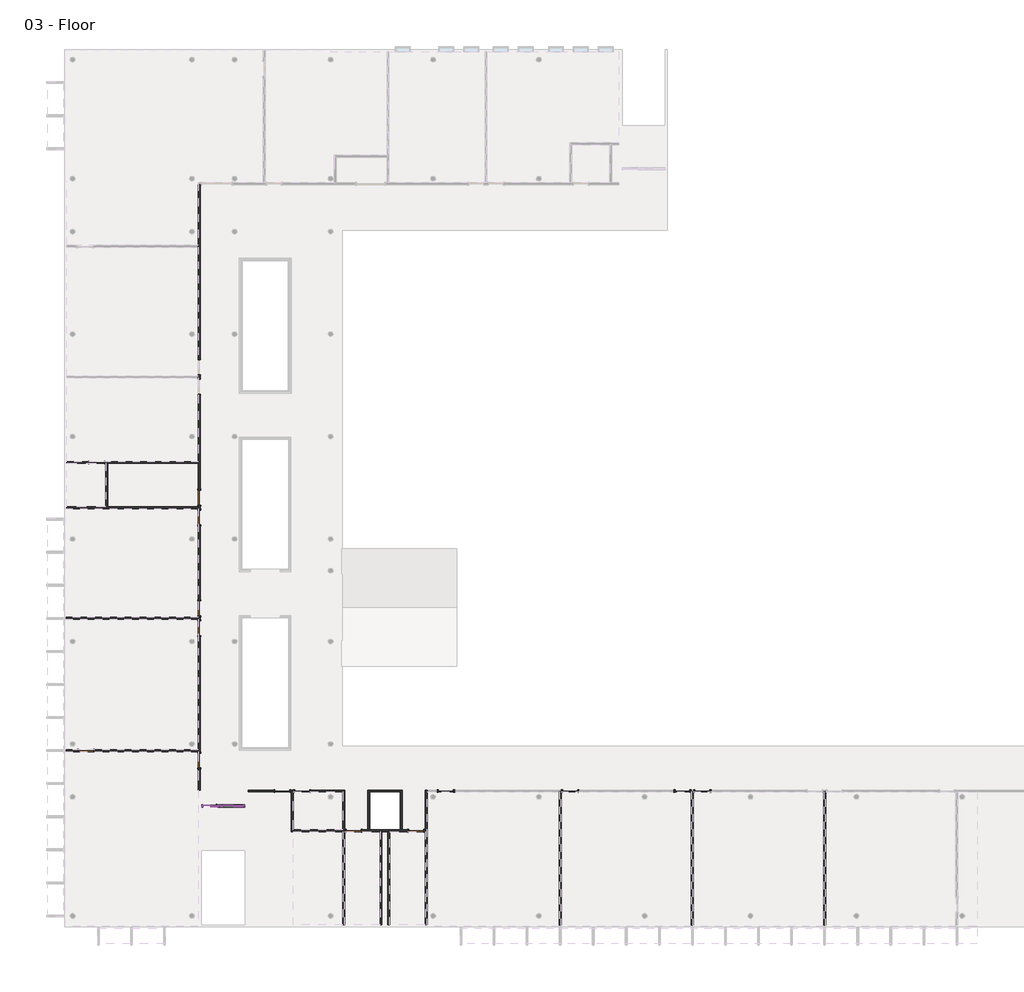
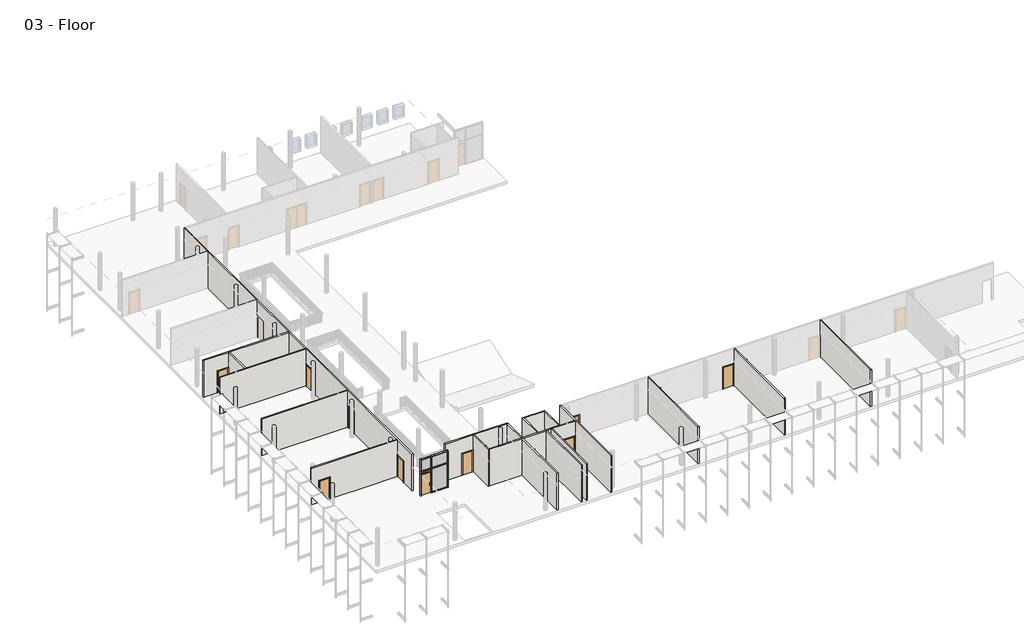
# One storey, part 1 of 4: 19 walls, 18 members, 16 doors, 4 plates.
"""IFC4 building model written with IfcOpenShell, lengths in millimetres."""

import ifcopenshell
import ifcopenshell.guid

model = None  # the IFC model being written
_history = None  # IfcOwnerHistory: only IFC2X3 demands one
_inside = {}  # id of a spatial element -> (the spatial element, [elements in it])
_under = {}  # id of a project, library or spatial element -> (it, [spatial elements below it])
_declared = {}  # id of a project -> (the project, [libraries it declares])
_typed = {}  # id of a type object -> (the type object, [elements of that type])
_made_of = {}  # id of a material, layer set ... -> (it, [elements and type objects made of it])


def new_model(schema):
    """Start an empty IFC model of exactly this schema.

    Asked for "IFC4X3", IfcOpenShell would pick the latest addendum, in which some entities
    have other attributes; the version numbers below select the first issue.
    IFC2X3 requires an IfcOwnerHistory on every rooted entity: one is made here for all.
    """
    global model, _history
    if schema == "IFC4X3":
        model = ifcopenshell.file(schema_version=(4, 3, 0, 0))
    else:
        model = ifcopenshell.file(schema=schema)
    _inside.clear()
    _under.clear()
    _declared.clear()
    _typed.clear()
    _made_of.clear()
    _history = None
    if model.schema == "IFC2X3":
        org = make("IfcOrganization", Name="unknown")
        user = make(
            "IfcPersonAndOrganization",
            ThePerson=make("IfcPerson", FamilyName="unknown"),
            TheOrganization=org,
        )
        app = make(
            "IfcApplication",
            ApplicationDeveloper=org,
            Version="unknown",
            ApplicationFullName="unknown",
            ApplicationIdentifier="unknown",
        )
        _history = make(
            "IfcOwnerHistory",
            OwningUser=user,
            OwningApplication=app,
            ChangeAction="ADDED",
            CreationDate=0,
        )
    return model


def make(cls, **values):
    """One entity of the class cls with the attributes given. An attribute that is None is left unset."""
    return model.create_entity(
        cls, **{name: value for name, value in values.items() if value is not None}
    )


def rooted(cls, **values):
    """An entity with a GlobalId (a new one), such as an element, a storey or a relation."""
    return make(cls, GlobalId=ifcopenshell.guid.new(), OwnerHistory=_history, **values)


def si_unit(unit_type, name, prefix=None):
    """IfcSIUnit, for example si_unit("LENGTHUNIT", "METRE", prefix="MILLI")."""
    return make("IfcSIUnit", UnitType=unit_type, Prefix=prefix, Name=name)


def assignment(units):
    """IfcUnitAssignment: the units of a project."""
    return None if units is None else make("IfcUnitAssignment", Units=units)


def point(xyz):
    """IfcCartesianPoint."""
    return None if xyz is None else make("IfcCartesianPoint", Coordinates=xyz)


def direction(xyz):
    """IfcDirection."""
    return None if xyz is None else make("IfcDirection", DirectionRatios=xyz)


def frame(location, z_axis=None, x_axis=None):
    """IfcAxis2Placement3D, a coordinate frame: its origin and axes. An axis left out is left unset."""
    return make(
        "IfcAxis2Placement3D",
        Location=point(location),
        Axis=direction(z_axis),
        RefDirection=direction(x_axis),
    )


def origin():
    """The frame at (0, 0, 0) with its axes left unset."""
    return frame((0.0, 0.0, 0.0))


def origin_with_axes():
    """The frame at (0, 0, 0) with the z axis (0, 0, 1) and the x axis (1, 0, 0) written out."""
    return frame((0.0, 0.0, 0.0), z_axis=(0.0, 0.0, 1.0), x_axis=(1.0, 0.0, 0.0))


def place(relative_to, where):
    """IfcLocalPlacement: puts the frame where relative to a parent placement (None: the world)."""
    return make(
        "IfcLocalPlacement", PlacementRelTo=relative_to, RelativePlacement=where
    )


def context(
    kind, dimensions, precision=None, world=None, true_north=None, identifier=None
):
    """IfcGeometricRepresentationContext, for example the 3D "Model" context."""
    return make(
        "IfcGeometricRepresentationContext",
        ContextIdentifier=identifier,
        ContextType=kind,
        CoordinateSpaceDimension=dimensions,
        Precision=precision,
        WorldCoordinateSystem=world,
        TrueNorth=true_north,
    )


def project(units=None, contexts=None):
    """IfcProject with its units and contexts."""
    return rooted(
        "IfcProject",
        Name="project",
        RepresentationContexts=contexts,
        UnitsInContext=assignment(units),
    )


def spatial(cls, under=None, at=None, **own):
    """A site, building, storey or space (cls), placed at a placement, below another one or the project."""
    s = rooted(cls, ObjectPlacement=at, **own)
    if under is not None:
        _under.setdefault(under.id(), (under, []))[1].append(s)
    return s


def polyline(points):
    """IfcPolyline through the points."""
    return make("IfcPolyline", Points=[point(p) for p in points])


def outline(outer, holes=None, kind="AREA"):
    """IfcArbitraryClosedProfileDef: a profile drawn as a closed curve; with holes, ...WithVoids."""
    if holes is None:
        return make("IfcArbitraryClosedProfileDef", ProfileType=kind, OuterCurve=outer)
    return make(
        "IfcArbitraryProfileDefWithVoids",
        ProfileType=kind,
        OuterCurve=outer,
        InnerCurves=holes,
    )


def extrude(swept, where, along, depth):
    """IfcExtrudedAreaSolid: the profile swept, set in the frame where, extruded along a direction by depth."""
    return make(
        "IfcExtrudedAreaSolid",
        SweptArea=swept,
        Position=where,
        ExtrudedDirection=direction(along),
        Depth=depth,
    )


def faces_of(points, faces, orient=None, outer=None):
    """IfcFace entities. A face is a list of loops; a loop is a list of indices into points, from 0.

    orient and outer hold one flag for each loop. By default every Orientation is true, the
    first loop of a face is its IfcFaceOuterBound and the others are IfcFaceBound.
    """
    made = []
    for i, loops in enumerate(faces):
        bounds = []
        for j, loop in enumerate(loops):
            is_outer = j == 0 if outer is None else outer[i][j]
            bounds.append(
                make(
                    "IfcFaceOuterBound" if is_outer else "IfcFaceBound",
                    Bound=make("IfcPolyLoop", Polygon=[points[k] for k in loop]),
                    Orientation=True if orient is None else orient[i][j],
                )
            )
        made.append(make("IfcFace", Bounds=bounds))
    return made


def faceted_brep(points, faces, orient=None, outer=None, voids=None):
    """IfcFacetedBrep: a solid bounded by flat faces; with voids (closed shells), ...WithVoids."""
    shared = [point(p) for p in points]
    hull = make("IfcClosedShell", CfsFaces=faces_of(shared, faces, orient, outer))
    if voids is None:
        return make("IfcFacetedBrep", Outer=hull)
    return make(
        "IfcFacetedBrepWithVoids",
        Outer=hull,
        Voids=[
            make(cls, CfsFaces=faces_of(shared, fs, o, b)) for cls, fs, o, b in voids
        ],
    )


def shape(context_of_items, identifier, shape_type, items):
    """IfcShapeRepresentation: the items that make up one representation, for example the "Body"."""
    return make(
        "IfcShapeRepresentation",
        ContextOfItems=context_of_items,
        RepresentationIdentifier=identifier,
        RepresentationType=shape_type,
        Items=items,
    )


def source(mapping_origin, context_of_items, identifier, shape_type, items):
    """IfcRepresentationMap: a shape defined once, which mapped items show again and again."""
    return make(
        "IfcRepresentationMap",
        MappingOrigin=mapping_origin,
        MappedRepresentation=shape(context_of_items, identifier, shape_type, items),
    )


def transform(
    local_origin,
    x_axis=None,
    y_axis=None,
    z_axis=None,
    scale=None,
    scale2=None,
    scale3=None,
    uniform=True,
):
    """IfcCartesianTransformationOperator3D, or its non-uniform kind. x_axis, y_axis, z_axis: its Axis1, 2, 3."""
    if uniform:
        return make(
            "IfcCartesianTransformationOperator3D",
            Axis1=direction(x_axis),
            Axis2=direction(y_axis),
            LocalOrigin=point(local_origin),
            Scale=scale,
            Axis3=direction(z_axis),
        )
    return make(
        "IfcCartesianTransformationOperator3DnonUniform",
        Axis1=direction(x_axis),
        Axis2=direction(y_axis),
        LocalOrigin=point(local_origin),
        Scale=scale,
        Axis3=direction(z_axis),
        Scale2=scale2,
        Scale3=scale3,
    )


def mapped(mapping_source, mapping_target):
    """IfcMappedItem: shows the shape of a source again, moved by a transform."""
    return make(
        "IfcMappedItem", MappingSource=mapping_source, MappingTarget=mapping_target
    )


def made_of(thing, what):
    """Note that an element or type object is made of a material, layer set ...; save() writes the relation."""
    if what is not None:
        _made_of.setdefault(what.id(), (what, []))[1].append(thing)
    return thing


def element(
    cls,
    number,
    at=None,
    inside=None,
    cuts=None,
    type_object=None,
    material=None,
    context=None,
    identifier="Body",
    shape_type=None,
    held_by="IfcProductDefinitionShape",
    body=None,
    shapes=None,
    **own,
):
    """One element of the class cls, such as IfcWall. Its Tag is "e" and its number.

    at: its placement. inside: the storey or other place that contains it. cuts: it is an
    opening in that element (IfcRelVoidsElement). A single representation is given by context,
    identifier, shape_type and body (its items); several are given by shapes. held_by: the class
    of the entity that holds the representations. save() writes the other relations.
    """
    e = rooted(cls, Tag="e%d" % number, ObjectPlacement=at, **own)
    if body is not None:
        shapes = [shape(context, identifier, shape_type, body)]
    if shapes is not None:
        e.Representation = make(held_by, Representations=shapes)
    if inside is not None:
        _inside.setdefault(inside.id(), (inside, []))[1].append(e)
    if cuts is not None:
        rooted(
            "IfcRelVoidsElement", RelatingBuildingElement=cuts, RelatedOpeningElement=e
        )
    if type_object is not None:
        _typed.setdefault(type_object.id(), (type_object, []))[1].append(e)
    return made_of(e, material)


def aggregate(whole, parts):
    """IfcRelAggregates: a whole, such as a stair, and the parts it consists of."""
    return rooted("IfcRelAggregates", RelatingObject=whole, RelatedObjects=parts)


def save(model, path):
    """Write the relations noted so far, then the file.

    IfcRelAggregates (storeys below a building ...), IfcRelContainedInSpatialStructure (elements
    in a storey), IfcRelDefinesByType, IfcRelAssociatesMaterial and IfcRelDeclares: one each for
    every whole, place, type object, material and project.
    """
    for whole, parts in _under.values():
        aggregate(whole, parts)
    for where, things in _inside.values():
        rooted(
            "IfcRelContainedInSpatialStructure",
            RelatedElements=things,
            RelatingStructure=where,
        )
    for kind, things in _typed.values():
        rooted("IfcRelDefinesByType", RelatedObjects=things, RelatingType=kind)
    for what, things in _made_of.values():
        rooted("IfcRelAssociatesMaterial", RelatedObjects=things, RelatingMaterial=what)
    for by, libraries in _declared.values():
        rooted("IfcRelDeclares", RelatingContext=by, RelatedDefinitions=libraries)
    model.write(path)


def curtain_wall_sgl_glass_curtain_wall_sgl_glass_c2d4b377(model_context):
    return source(origin(), model_context, "Body", "SweptSolid", [
        extrude(outline(polyline([(-355.6, 12.7), (-355.6, -38.1), (-381.0, -38.1), (-381.0, 12.7), (-355.6, 12.7)])), frame((0.0, 0.0, 762.0), z_axis=(0.0, 0.0, 1.0), x_axis=(1.0, 0.0, 0.0)), (0.0, 0.0, 1.0), 228.6),
        extrude(outline(polyline([(-381.0, -101.6), (-381.0, -50.8), (-355.6, -50.8), (-355.6, -101.6), (-381.0, -101.6)])), frame((0.0, 0.0, 762.0), z_axis=(0.0, 0.0, 1.0), x_axis=(1.0, 0.0, 0.0)), (0.0, 0.0, 1.0), 228.6),
        extrude(outline(polyline([(457.2, -50.8), (-457.2, -50.8), (-457.2, -38.1), (457.2, -38.1), (457.2, -50.8)])), origin_with_axes(), (0.0, 0.0, 1.0), 2133.6),
    ])


def door_305aa2a5(model_context):
    return source(origin(), model_context, "Body", "SweptSolid", [
        extrude(outline(polyline([(2209.8, -533.4), (0.0, -533.4), (0.0, -457.2), (2133.6, -457.2), (2133.6, 457.2), (0.0, 457.2), (0.0, 533.4), (2209.8, 533.4), (2209.8, -533.4)])), frame((0.0, -82.55, 0.0), z_axis=(0.0, 1.0, 0.0), x_axis=(0.0, 0.0, 1.0)), (0.0, 0.0, 1.0), 25.4),
        extrude(outline(polyline([(2209.8, 533.4), (2209.8, -533.4), (0.0, -533.4), (0.0, -457.2), (2133.6, -457.2), (2133.6, 457.2), (0.0, 457.2), (0.0, 533.4), (2209.8, 533.4)])), frame((0.0, 57.15, 0.0), z_axis=(0.0, 1.0, 0.0), x_axis=(0.0, 0.0, 1.0)), (0.0, 0.0, 1.0), 25.4),
        extrude(outline(polyline([(457.2, -6.35), (457.2, -57.15), (-457.2, -57.15), (-457.2, -6.35), (457.2, -6.35)])), origin_with_axes(), (0.0, 0.0, 1.0), 2133.6),
    ])


def door_e5f9f3c4(model_context):
    return source(origin(), model_context, "Body", "SweptSolid", [
        extrude(outline(polyline([(2209.8, -533.4), (0.0, -533.4), (0.0, -457.2), (2133.6, -457.2), (2133.6, 457.2), (0.0, 457.2), (0.0, 533.4), (2209.8, 533.4), (2209.8, -533.4)])), frame((0.0, 57.15, 0.0), z_axis=(0.0, 1.0, 0.0), x_axis=(0.0, 0.0, 1.0)), (0.0, 0.0, 1.0), 25.4),
        extrude(outline(polyline([(2209.8, 533.4), (2209.8, -533.4), (0.0, -533.4), (0.0, -457.2), (2133.6, -457.2), (2133.6, 457.2), (0.0, 457.2), (0.0, 533.4), (2209.8, 533.4)])), frame((0.0, -82.55, 0.0), z_axis=(0.0, 1.0, 0.0), x_axis=(0.0, 0.0, 1.0)), (0.0, 0.0, 1.0), 25.4),
        extrude(outline(polyline([(457.2, 6.35), (-457.2, 6.35), (-457.2, 57.15), (457.2, 57.15), (457.2, 6.35)])), origin_with_axes(), (0.0, 0.0, 1.0), 2133.6),
    ])


def member_2b49869a(model_context):
    return source(origin(), model_context, "Body", "SweptSolid", [
        extrude(outline(polyline([(31.75, 63.5), (31.75, -63.5), (-31.75, -63.5), (-31.75, 63.5), (31.75, 63.5)])), frame((0.0, 0.0, -1219.2), z_axis=(0.0, 0.0, 1.0), x_axis=(1.0, 0.0, 0.0)), (0.0, 0.0, 1.0), 1219.2),
    ])


def member_75074519(model_context):
    return source(origin(), model_context, "Body", "SweptSolid", [
        extrude(outline(polyline([(0.0, 63.5), (0.0, -63.5), (-63.5, -63.5), (-63.5, 63.5), (0.0, 63.5)])), frame((0.0, 0.0, -1219.2), z_axis=(0.0, 0.0, 1.0), x_axis=(1.0, 0.0, 0.0)), (0.0, 0.0, 1.0), 1219.2),
    ])


def member_6186cc23(model_context):
    return source(origin(), model_context, "Body", "SweptSolid", [
        extrude(outline(polyline([(31.75, 63.5), (31.75, -63.5), (-31.75, -63.5), (-31.75, 63.5), (31.75, 63.5)])), frame((0.0, 0.0, -2165.35), z_axis=(0.0, 0.0, 1.0), x_axis=(1.0, 0.0, 0.0)), (0.0, 0.0, 1.0), 2165.35),
    ])


def member_5d67b9fc(model_context):
    return source(origin(), model_context, "Body", "SweptSolid", [
        extrude(outline(polyline([(31.75, 63.5), (31.75, -63.5), (-31.75, -63.5), (-31.75, 63.5), (31.75, 63.5)])), frame((0.0, 0.0, -273.05), z_axis=(0.0, 0.0, 1.0), x_axis=(1.0, 0.0, 0.0)), (0.0, 0.0, 1.0), 273.05),
    ])


def member_c327c56d(model_context):
    return source(origin(), model_context, "Body", "SweptSolid", [
        extrude(outline(polyline([(0.0, 63.5), (0.0, -63.5), (-63.5, -63.5), (-63.5, 63.5), (0.0, 63.5)])), frame((0.0, 0.0, -273.05), z_axis=(0.0, 0.0, 1.0), x_axis=(1.0, 0.0, 0.0)), (0.0, 0.0, 1.0), 273.05),
    ])


def member_a50b3cda(model_context):
    return source(origin(), model_context, "Body", "SweptSolid", [
        extrude(outline(polyline([(0.0, 63.5), (0.0, -63.5), (-63.5, -63.5), (-63.5, 63.5), (0.0, 63.5)])), frame((0.0, 0.0, -2165.35), z_axis=(0.0, 0.0, 1.0), x_axis=(1.0, 0.0, 0.0)), (0.0, 0.0, 1.0), 2165.35),
    ])


def member_410c6227(model_context):
    return source(origin(), model_context, "Body", "SweptSolid", [
        extrude(outline(polyline([(31.75, 63.5), (31.75, -63.5), (-31.75, -63.5), (-31.75, 63.5), (31.75, 63.5)])), frame((0.0, 0.0, -914.4), z_axis=(0.0, 0.0, 1.0), x_axis=(1.0, 0.0, 0.0)), (0.0, 0.0, 1.0), 914.4),
    ])


def member_73c23c35(model_context):
    return source(origin(), model_context, "Body", "SweptSolid", [
        extrude(outline(polyline([(0.0, 63.5), (0.0, -63.5), (-63.5, -63.5), (-63.5, 63.5), (0.0, 63.5)])), frame((0.0, 0.0, -914.4), z_axis=(0.0, 0.0, 1.0), x_axis=(1.0, 0.0, 0.0)), (0.0, 0.0, 1.0), 914.4),
    ])


def member_59c53a79(model_context):
    return source(origin(), model_context, "Body", "SweptSolid", [
        extrude(outline(polyline([(0.0, 63.5), (0.0, -63.5), (-63.5, -63.5), (-63.5, 63.5), (0.0, 63.5)])), frame((0.0, 0.0, -1245.39375), z_axis=(0.0, 0.0, 1.0), x_axis=(1.0, 0.0, 0.0)), (0.0, 0.0, 1.0), 1245.39375),
    ])


def member_c46932f7(model_context):
    return source(origin(), model_context, "Body", "SweptSolid", [
        extrude(outline(polyline([(31.75, 63.5), (31.75, -63.5), (-31.75, -63.5), (-31.75, 63.5), (31.75, 63.5)])), frame((0.0, 0.0, -1245.39375), z_axis=(0.0, 0.0, 1.0), x_axis=(1.0, 0.0, 0.0)), (0.0, 0.0, 1.0), 1245.39375),
    ])


def member_40e8ea34(model_context):
    return source(origin(), model_context, "Body", "SweptSolid", [
        extrude(outline(polyline([(31.75, 63.5), (31.75, -63.5), (-31.75, -63.5), (-31.75, 63.5), (31.75, 63.5)])), frame((0.0, 0.0, -267.49375), z_axis=(0.0, 0.0, 1.0), x_axis=(1.0, 0.0, 0.0)), (0.0, 0.0, 1.0), 267.49375),
    ])


def member_f5b3432e(model_context):
    return source(origin(), model_context, "Body", "SweptSolid", [
        extrude(outline(polyline([(0.0, 63.5), (0.0, -63.5), (-63.5, -63.5), (-63.5, 63.5), (0.0, 63.5)])), frame((0.0, 0.0, -267.49375), z_axis=(0.0, 0.0, 1.0), x_axis=(1.0, 0.0, 0.0)), (0.0, 0.0, 1.0), 267.49375),
    ])


def system_panel_glazed_8dc8626f(model_context):
    return source(origin(), model_context, "Body", "SweptSolid", [
        extrude(outline(polyline([(457.2, -44.45), (-457.2, -44.45), (-457.2, -19.05), (457.2, -19.05), (457.2, -44.45)])), origin_with_axes(), (0.0, 0.0, 1.0), 209.55),
    ])


def system_panel_glazed_2e5f6ce9(model_context):
    return source(origin(), model_context, "Body", "SweptSolid", [
        extrude(outline(polyline([(457.2, -44.45), (-457.2, -44.45), (-457.2, -19.05), (457.2, -19.05), (457.2, -44.45)])), origin_with_axes(), (0.0, 0.0, 1.0), 1123.95),
    ])


def system_panel_glazed_8d3e4aee(model_context):
    return source(origin(), model_context, "Body", "SweptSolid", [
        extrude(outline(polyline([(0.0, -756.44375), (0.0, 488.95), (0.0, 756.44375), (2101.85, 756.44375), (2343.15, 756.44375), (2343.15, 488.95), (2343.15, -756.44375), (2101.85, -756.44375), (0.0, -756.44375)])), frame((0.0, -44.45, 0.0), z_axis=(0.0, 1.0, 0.0), x_axis=(0.0, 0.0, 1.0)), (0.0, 0.0, 1.0), 25.4),
    ])


def system_panel_glazed_fabe228a(model_context):
    return source(origin(), model_context, "Body", "SweptSolid", [
        extrude(outline(polyline([(0.0, -756.44375), (0.0, 488.95), (0.0, 756.44375), (1123.95, 756.44375), (1123.95, 488.95), (1123.95, -756.44375), (0.0, -756.44375)])), frame((0.0, -44.45, 0.0), z_axis=(0.0, 1.0, 0.0), x_axis=(0.0, 0.0, 1.0)), (0.0, 0.0, 1.0), 25.4),
    ])


model = new_model("IFC4")

# Units and contexts
model_context = context("Model", 3, world=origin())
ifc_project = project(units=[si_unit("LENGTHUNIT", "METRE", prefix="MILLI")], contexts=[model_context])

# Site, building, storey
site = spatial("IfcSite", under=ifc_project)
building = spatial("IfcBuilding", under=site)
storey = spatial("IfcBuildingStorey", under=building, Name="03 - Floor", Elevation=7315.2)

# Doors
placement = place(None, origin())
curtain_wall_sgl_glass_curtain_wall_sgl_glass_shape = curtain_wall_sgl_glass_curtain_wall_sgl_glass_c2d4b377(model_context)
element("IfcDoor", 1, ObjectType="Curtain Wall Sgl Glass : Curtain Wall Sgl Glass", at=placement, inside=storey, context=model_context, shape_type="MappedRepresentation", body=[
    mapped(curtain_wall_sgl_glass_curtain_wall_sgl_glass_shape, transform((9097.2957476, 7356.4, 7315.2), x_axis=(-1.0, 0.0, 0.0), y_axis=(0.0, -1.0, 0.0), z_axis=(0.0, 0.0, 1.0))),
])
door_shape = door_305aa2a5(model_context)
element("IfcDoor", 2, ObjectType="Single-Flush : 36\" x 84\"", at=placement, inside=storey, context=model_context, shape_type="MappedRepresentation", body=[
    mapped(door_shape, transform((21743.3207476, 5832.4, 7315.2), x_axis=(1.0, 0.0, 0.0), y_axis=(0.0, 1.0, 0.0), z_axis=(0.0, 0.0, 1.0))),
])
element("IfcDoor", 3, ObjectType="Single-Flush : 36\" x 84\"", at=placement, inside=storey, context=model_context, shape_type="MappedRepresentation", body=[
    mapped(door_shape, transform((2109.1207476, 28463.8, 7315.2), x_axis=(1.0, 0.0, 0.0), y_axis=(0.0, 1.0, 0.0), z_axis=(0.0, 0.0, 1.0))),
])
element("IfcDoor", 4, ObjectType="Single-Flush : 36\" x 84\"", at=placement, inside=storey, context=model_context, shape_type="MappedRepresentation", body=[
    mapped(door_shape, transform((8414.6707476, 26304.8, 7315.2), x_axis=(0.0, -1.0, 0.0), y_axis=(1.0, 0.0, 0.0), z_axis=(0.0, 0.0, 1.0))),
])
element("IfcDoor", 5, ObjectType="Single-Flush : 36\" x 84\"", at=placement, inside=storey, context=model_context, shape_type="MappedRepresentation", body=[
    mapped(door_shape, transform((8414.6707476, 19497.6, 7315.2), x_axis=(0.0, -1.0, 0.0), y_axis=(1.0, 0.0, 0.0), z_axis=(0.0, 0.0, 1.0))),
])
element("IfcDoor", 6, ObjectType="Single-Flush : 36\" x 84\"", at=placement, inside=storey, context=model_context, shape_type="MappedRepresentation", body=[
    mapped(door_shape, transform((13513.7207476, 8277.15, 7315.2), x_axis=(1.0, 0.0, 0.0), y_axis=(0.0, 1.0, 0.0), z_axis=(0.0, 0.0, 1.0))),
])
element("IfcDoor", 7, ObjectType="Single-Flush : 36\" x 84\"", at=placement, inside=storey, context=model_context, shape_type="MappedRepresentation", body=[
    mapped(door_shape, transform((38113.6207476, 8277.15, 7315.2), x_axis=(1.0, 0.0, 0.0), y_axis=(0.0, 1.0, 0.0), z_axis=(0.0, 0.0, 1.0))),
])
door_2_shape = door_e5f9f3c4(model_context)
element("IfcDoor", 8, ObjectType="Single-Flush : 36\" x 84\"", at=placement, inside=storey, context=model_context, shape_type="MappedRepresentation", body=[
    mapped(door_2_shape, transform((17907.9207476, 5832.4, 7315.2), x_axis=(-1.0, 0.0, 0.0), y_axis=(0.0, -1.0, 0.0), z_axis=(0.0, 0.0, 1.0))),
])
element("IfcDoor", 9, ObjectType="Single-Flush : 36\" x 84\"", at=placement, inside=storey, context=model_context, shape_type="MappedRepresentation", body=[
    mapped(door_2_shape, transform((8414.6707476, 25085.6, 7315.2), x_axis=(0.0, 1.0, 0.0), y_axis=(-1.0, 0.0, 0.0), z_axis=(0.0, 0.0, 1.0))),
])
element("IfcDoor", 10, ObjectType="Single-Flush : 36\" x 84\"", at=placement, inside=storey, context=model_context, shape_type="MappedRepresentation", body=[
    mapped(door_2_shape, transform((8414.6707476, 18278.4, 7315.2), x_axis=(0.0, 1.0, 0.0), y_axis=(-1.0, 0.0, 0.0), z_axis=(0.0, 0.0, 1.0))),
])
element("IfcDoor", 11, ObjectType="Single-Flush : 36\" x 84\"", at=placement, inside=storey, context=model_context, shape_type="MappedRepresentation", body=[
    mapped(door_2_shape, transform((1448.7207476, 10760.0, 7315.2), x_axis=(-1.0, 0.0, 0.0), y_axis=(0.0, -1.0, 0.0), z_axis=(0.0, 0.0, 1.0))),
])
element("IfcDoor", 12, ObjectType="Single-Flush : 36\" x 84\"", at=placement, inside=storey, context=model_context, shape_type="MappedRepresentation", body=[
    mapped(door_2_shape, transform((8414.6707476, 10150.4, 7315.2), x_axis=(0.0, 1.0, 0.0), y_axis=(-1.0, 0.0, 0.0), z_axis=(0.0, 0.0, 1.0))),
])
element("IfcDoor", 13, ObjectType="Single-Flush : 36\" x 84\"", at=placement, inside=storey, context=model_context, shape_type="MappedRepresentation", body=[
    mapped(door_2_shape, transform((14732.9207476, 8277.15, 7315.2), x_axis=(-1.0, 0.0, 0.0), y_axis=(0.0, -1.0, 0.0), z_axis=(0.0, 0.0, 1.0))),
])
element("IfcDoor", 14, ObjectType="Single-Flush : 36\" x 84\"", at=placement, inside=storey, context=model_context, shape_type="MappedRepresentation", body=[
    mapped(door_2_shape, transform((23572.1207476, 8277.15, 7315.2), x_axis=(-1.0, 0.0, 0.0), y_axis=(0.0, -1.0, 0.0), z_axis=(0.0, 0.0, 1.0))),
])
element("IfcDoor", 15, ObjectType="Single-Flush : 36\" x 84\"", at=placement, inside=storey, context=model_context, shape_type="MappedRepresentation", body=[
    mapped(door_2_shape, transform((31204.8207476, 8277.15, 7315.2), x_axis=(-1.0, 0.0, 0.0), y_axis=(0.0, -1.0, 0.0), z_axis=(0.0, 0.0, 1.0))),
])
element("IfcDoor", 16, ObjectType="Single-Flush : 36\" x 84\"", at=placement, inside=storey, context=model_context, shape_type="MappedRepresentation", body=[
    mapped(door_2_shape, transform((39332.8207476, 8277.15, 7315.2), x_axis=(-1.0, 0.0, 0.0), y_axis=(0.0, -1.0, 0.0), z_axis=(0.0, 0.0, 1.0))),
])

# Members
member_shape = member_2b49869a(model_context)
element("IfcMember", 17, ObjectType="Rectangular Mullion : 2.5\" x 5\" rectangular", at=placement, inside=storey, context=model_context, shape_type="MappedRepresentation", body=[
    mapped(member_shape, transform((9586.2457476, 7356.4, 9753.6), x_axis=(-1.0, 0.0, 0.0), y_axis=(0.0, 1.0, 0.0), z_axis=(0.0, 0.0, -1.0))),
])
member_2_shape = member_75074519(model_context)
element("IfcMember", 18, ObjectType="Rectangular Mullion : 2.5\" x 5\" rectangular", at=placement, inside=storey, context=model_context, shape_type="MappedRepresentation", body=[
    mapped(member_2_shape, transform((11194.3832476, 7356.4, 10972.8), x_axis=(1.0, 0.0, 0.0), y_axis=(0.0, 1.0, 0.0), z_axis=(0.0, 0.0, 1.0))),
])
element("IfcMember", 19, ObjectType="Rectangular Mullion : 2.5\" x 5\" rectangular", at=placement, inside=storey, context=model_context, shape_type="MappedRepresentation", body=[
    mapped(member_2_shape, transform((8576.5957476, 7356.4, 9753.6), x_axis=(-1.0, 0.0, 0.0), y_axis=(0.0, 1.0, 0.0), z_axis=(0.0, 0.0, -1.0))),
])
member_3_shape = member_6186cc23(model_context)
element("IfcMember", 20, ObjectType="Rectangular Mullion : 2.5\" x 5\" rectangular", at=placement, inside=storey, context=model_context, shape_type="MappedRepresentation", body=[
    mapped(member_3_shape, transform((9586.2457476, 7356.4, 7315.2), x_axis=(-1.0, 0.0, 0.0), y_axis=(0.0, 1.0, 0.0), z_axis=(0.0, 0.0, -1.0))),
])
member_4_shape = member_5d67b9fc(model_context)
element("IfcMember", 21, ObjectType="Rectangular Mullion : 2.5\" x 5\" rectangular", at=placement, inside=storey, context=model_context, shape_type="MappedRepresentation", body=[
    mapped(member_4_shape, transform((9586.2457476, 7356.4, 9480.55), x_axis=(-1.0, 0.0, 0.0), y_axis=(0.0, 1.0, 0.0), z_axis=(0.0, 0.0, -1.0))),
])
member_5_shape = member_c327c56d(model_context)
element("IfcMember", 22, ObjectType="Rectangular Mullion : 2.5\" x 5\" rectangular", at=placement, inside=storey, context=model_context, shape_type="MappedRepresentation", body=[
    mapped(member_5_shape, transform((11194.3832476, 7356.4, 9753.6), x_axis=(1.0, 0.0, 0.0), y_axis=(0.0, 1.0, 0.0), z_axis=(0.0, 0.0, 1.0))),
])
member_6_shape = member_a50b3cda(model_context)
element("IfcMember", 23, ObjectType="Rectangular Mullion : 2.5\" x 5\" rectangular", at=placement, inside=storey, context=model_context, shape_type="MappedRepresentation", body=[
    mapped(member_6_shape, transform((11194.3832476, 7356.4, 9480.55), x_axis=(1.0, 0.0, 0.0), y_axis=(0.0, 1.0, 0.0), z_axis=(0.0, 0.0, 1.0))),
])
member_7_shape = member_410c6227(model_context)
element("IfcMember", 24, ObjectType="Rectangular Mullion : 2.5\" x 5\" rectangular", at=placement, inside=storey, context=model_context, shape_type="MappedRepresentation", body=[
    mapped(member_7_shape, transform((8640.0957476, 7356.4, 9753.6), x_axis=(0.0, 0.0, 1.0), y_axis=(0.0, 1.0, 0.0), z_axis=(-1.0, 0.0, 0.0))),
])
element("IfcMember", 25, ObjectType="Rectangular Mullion : 2.5\" x 5\" rectangular", at=placement, inside=storey, context=model_context, shape_type="MappedRepresentation", body=[
    mapped(member_7_shape, transform((8640.0957476, 7356.4, 9480.55), x_axis=(0.0, 0.0, 1.0), y_axis=(0.0, 1.0, 0.0), z_axis=(-1.0, 0.0, 0.0))),
])
member_8_shape = member_73c23c35(model_context)
element("IfcMember", 26, ObjectType="Rectangular Mullion : 2.5\" x 5\" rectangular", at=placement, inside=storey, context=model_context, shape_type="MappedRepresentation", body=[
    mapped(member_8_shape, transform((8640.0957476, 7356.4, 10972.8), x_axis=(0.0, 0.0, 1.0), y_axis=(0.0, 1.0, 0.0), z_axis=(-1.0, 0.0, 0.0))),
])
element("IfcMember", 27, ObjectType="Rectangular Mullion : 2.5\" x 5\" rectangular", at=placement, inside=storey, context=model_context, shape_type="MappedRepresentation", body=[
    mapped(member_6_shape, transform((8576.5957476, 7356.4, 7315.2), x_axis=(-1.0, 0.0, 0.0), y_axis=(0.0, 1.0, 0.0), z_axis=(0.0, 0.0, -1.0))),
])
element("IfcMember", 28, ObjectType="Rectangular Mullion : 2.5\" x 5\" rectangular", at=placement, inside=storey, context=model_context, shape_type="MappedRepresentation", body=[
    mapped(member_5_shape, transform((8576.5957476, 7356.4, 9480.55), x_axis=(-1.0, 0.0, 0.0), y_axis=(0.0, 1.0, 0.0), z_axis=(0.0, 0.0, -1.0))),
])
member_9_shape = member_59c53a79(model_context)
element("IfcMember", 29, ObjectType="Rectangular Mullion : 2.5\" x 5\" rectangular", at=placement, inside=storey, context=model_context, shape_type="MappedRepresentation", body=[
    mapped(member_9_shape, transform((11130.8832476, 7356.4, 7315.2), x_axis=(0.0, 0.0, -1.0), y_axis=(0.0, 1.0, 0.0), z_axis=(1.0, 0.0, 0.0))),
])
member_10_shape = member_c46932f7(model_context)
element("IfcMember", 30, ObjectType="Rectangular Mullion : 2.5\" x 5\" rectangular", at=placement, inside=storey, context=model_context, shape_type="MappedRepresentation", body=[
    mapped(member_10_shape, transform((9885.4894976, 7356.4, 9753.6), x_axis=(0.0, 0.0, 1.0), y_axis=(0.0, 1.0, 0.0), z_axis=(-1.0, 0.0, 0.0))),
])
element("IfcMember", 31, ObjectType="Rectangular Mullion : 2.5\" x 5\" rectangular", at=placement, inside=storey, context=model_context, shape_type="MappedRepresentation", body=[
    mapped(member_9_shape, transform((9885.4894976, 7356.4, 10972.8), x_axis=(0.0, 0.0, 1.0), y_axis=(0.0, 1.0, 0.0), z_axis=(-1.0, 0.0, 0.0))),
])
member_11_shape = member_40e8ea34(model_context)
element("IfcMember", 32, ObjectType="Rectangular Mullion : 2.5\" x 5\" rectangular", at=placement, inside=storey, context=model_context, shape_type="MappedRepresentation", body=[
    mapped(member_11_shape, transform((9617.9957476, 7356.4, 9753.6), x_axis=(0.0, 0.0, 1.0), y_axis=(0.0, 1.0, 0.0), z_axis=(-1.0, 0.0, 0.0))),
])
member_12_shape = member_f5b3432e(model_context)
element("IfcMember", 33, ObjectType="Rectangular Mullion : 2.5\" x 5\" rectangular", at=placement, inside=storey, context=model_context, shape_type="MappedRepresentation", body=[
    mapped(member_12_shape, transform((9617.9957476, 7356.4, 10972.8), x_axis=(0.0, 0.0, 1.0), y_axis=(0.0, 1.0, 0.0), z_axis=(-1.0, 0.0, 0.0))),
])
element("IfcMember", 34, ObjectType="Rectangular Mullion : 2.5\" x 5\" rectangular", at=placement, inside=storey, context=model_context, shape_type="MappedRepresentation", body=[
    mapped(member_12_shape, transform((9885.4894976, 7356.4, 7315.2), x_axis=(0.0, 0.0, -1.0), y_axis=(0.0, 1.0, 0.0), z_axis=(1.0, 0.0, 0.0))),
])

# Plates
system_panel_glazed_shape = system_panel_glazed_8dc8626f(model_context)
element("IfcPlate", 35, ObjectType="System Panel : Glazed", at=placement, inside=storey, context=model_context, shape_type="MappedRepresentation", body=[
    mapped(system_panel_glazed_shape, transform((9097.2957476, 7356.4, 9512.3), x_axis=(-1.0, 0.0, 0.0), y_axis=(0.0, -1.0, 0.0), z_axis=(0.0, 0.0, 1.0))),
])
system_panel_glazed_2_shape = system_panel_glazed_2e5f6ce9(model_context)
element("IfcPlate", 36, ObjectType="System Panel : Glazed", at=placement, inside=storey, context=model_context, shape_type="MappedRepresentation", body=[
    mapped(system_panel_glazed_2_shape, transform((9097.2957476, 7356.4, 9785.35), x_axis=(-1.0, 0.0, 0.0), y_axis=(0.0, -1.0, 0.0), z_axis=(0.0, 0.0, 1.0))),
])
system_panel_glazed_3_shape = system_panel_glazed_8d3e4aee(model_context)
element("IfcPlate", 37, ObjectType="System Panel : Glazed", at=placement, inside=storey, context=model_context, shape_type="MappedRepresentation", body=[
    mapped(system_panel_glazed_3_shape, transform((10374.4394976, 7356.4, 7378.7), x_axis=(-1.0, 0.0, 0.0), y_axis=(0.0, -1.0, 0.0), z_axis=(0.0, 0.0, 1.0))),
])
system_panel_glazed_4_shape = system_panel_glazed_fabe228a(model_context)
element("IfcPlate", 38, ObjectType="System Panel : Glazed", at=placement, inside=storey, context=model_context, shape_type="MappedRepresentation", body=[
    mapped(system_panel_glazed_4_shape, transform((10374.4394976, 7356.4, 9785.35), x_axis=(-1.0, 0.0, 0.0), y_axis=(0.0, -1.0, 0.0), z_axis=(0.0, 0.0, 1.0))),
])

# Walls
element("IfcWall", 39, ObjectType="Typ. Partition Wall", at=placement, inside=storey, context=model_context, shape_type="Brep", body=[
    faceted_brep([(8357.5207476, 17821.2, 7315.2), (8357.5207476, 10817.15, 7315.2), (8357.5207476, 10702.85, 7315.2), (8357.5207476, 10607.6, 7315.2), (8357.5207476, 10607.6, 9448.8), (8357.5207476, 9693.2, 9448.8), (8357.5207476, 9693.2, 7315.2), (8357.5207476, 8334.3, 7315.2), (8357.5207476, 8334.3, 10972.8), (8357.5207476, 10702.85, 10972.8), (8357.5207476, 10817.15, 10972.8), (8357.5207476, 18830.85, 10972.8), (8357.5207476, 18945.15, 10972.8), (8357.5207476, 25638.05, 10972.8), (8357.5207476, 25752.35, 10972.8), (8357.5207476, 28406.65, 10972.8), (8357.5207476, 28520.95, 10972.8), (8357.5207476, 33664.45, 10972.8), (8357.5207476, 33778.75, 10972.8), (8357.5207476, 41690.85, 10972.8), (8357.5207476, 41805.15, 10972.8), (8357.5207476, 45545.3, 10972.8), (8357.5207476, 45545.3, 7315.2), (8357.5207476, 41805.15, 7315.2), (8357.5207476, 41690.85, 7315.2), (8357.5207476, 34788.4, 7315.2), (8357.5207476, 34788.4, 9448.8), (8357.5207476, 33874.0, 9448.8), (8357.5207476, 33874.0, 7315.2), (8357.5207476, 33778.75, 7315.2), (8357.5207476, 33664.45, 7315.2), (8357.5207476, 33569.2, 7315.2), (8357.5207476, 33569.2, 9448.8), (8357.5207476, 32654.8, 9448.8), (8357.5207476, 32654.8, 7315.2), (8357.5207476, 28520.95, 7315.2), (8357.5207476, 28406.65, 7315.2), (8357.5207476, 26762.0, 7315.2), (8357.5207476, 26762.0, 9448.8), (8357.5207476, 25847.6, 9448.8), (8357.5207476, 25847.6, 7315.2), (8357.5207476, 25752.35, 7315.2), (8357.5207476, 25638.05, 7315.2), (8357.5207476, 25542.8, 7315.2), (8357.5207476, 25542.8, 9448.8), (8357.5207476, 24628.4, 9448.8), (8357.5207476, 24628.4, 7315.2), (8357.5207476, 19954.8, 7315.2), (8357.5207476, 19954.8, 9448.8), (8357.5207476, 19040.4, 9448.8), (8357.5207476, 19040.4, 7315.2), (8357.5207476, 18945.15, 7315.2), (8357.5207476, 18830.85, 7315.2), (8357.5207476, 18735.6, 7315.2), (8357.5207476, 18735.6, 9448.8), (8357.5207476, 17821.2, 9448.8), (8471.8207476, 10607.6, 9448.8), (8471.8207476, 10607.6, 7315.2), (8471.8207476, 17821.2, 7315.2), (8471.8207476, 17821.2, 9448.8), (8471.8207476, 18735.6, 9448.8), (8471.8207476, 18735.6, 7315.2), (8471.8207476, 19040.4, 7315.2), (8471.8207476, 19040.4, 9448.8), (8471.8207476, 19954.8, 9448.8), (8471.8207476, 19954.8, 7315.2), (8471.8207476, 24628.4, 7315.2), (8471.8207476, 24628.4, 9448.8), (8471.8207476, 25542.8, 9448.8), (8471.8207476, 25542.8, 7315.2), (8471.8207476, 25847.6, 7315.2), (8471.8207476, 25847.6, 9448.8), (8471.8207476, 26762.0, 9448.8), (8471.8207476, 26762.0, 7315.2), (8471.8207476, 32654.8, 7315.2), (8471.8207476, 32654.8, 9448.8), (8471.8207476, 33569.2, 9448.8), (8471.8207476, 33569.2, 7315.2), (8471.8207476, 33874.0, 7315.2), (8471.8207476, 33874.0, 9448.8), (8471.8207476, 34788.4, 9448.8), (8471.8207476, 34788.4, 7315.2), (8471.8207476, 45545.3, 7315.2), (8471.8207476, 45545.3, 10972.8), (8471.8207476, 8334.3, 10972.8), (8471.8207476, 8334.3, 7315.2), (8471.8207476, 9693.2, 7315.2), (8471.8207476, 9693.2, 9448.8)], [[[0, 1, 2, 3, 4, 5, 6, 7, 8, 9, 10, 11, 12, 13, 14, 15, 16, 17, 18, 19, 20, 21, 22, 23, 24, 25, 26, 27, 28, 29, 30, 31, 32, 33, 34, 35, 36, 37, 38, 39, 40, 41, 42, 43, 44, 45, 46, 47, 48, 49, 50, 51, 52, 53, 54, 55]], [[56, 57, 58, 59, 60, 61, 62, 63, 64, 65, 66, 67, 68, 69, 70, 71, 72, 73, 74, 75, 76, 77, 78, 79, 80, 81, 82, 83, 84, 85, 86, 87]], [[78, 77, 31, 30, 29, 28]], [[25, 24, 23, 22, 82, 81]], [[70, 69, 43, 42, 41, 40]], [[37, 36, 35, 34, 74, 73]], [[62, 61, 53, 52, 51, 50]], [[47, 46, 66, 65]], [[58, 57, 3, 2, 1, 0]], [[86, 85, 7, 6]], [[8, 7, 85, 84]], [[21, 20, 19, 18, 17, 16, 15, 14, 13, 12, 11, 10, 9, 8, 84, 83]], [[22, 21, 83, 82]], [[79, 78, 28, 27]], [[80, 79, 27, 26]], [[81, 80, 26, 25]], [[32, 31, 77, 76]], [[33, 32, 76, 75]], [[34, 33, 75, 74]], [[71, 70, 40, 39]], [[72, 71, 39, 38]], [[73, 72, 38, 37]], [[44, 43, 69, 68]], [[45, 44, 68, 67]], [[46, 45, 67, 66]], [[63, 62, 50, 49]], [[64, 63, 49, 48]], [[65, 64, 48, 47]], [[54, 53, 61, 60]], [[55, 54, 60, 59]], [[0, 55, 59, 58]], [[4, 3, 57, 56]], [[5, 4, 56, 87]], [[6, 5, 87, 86]]]),
])
element("IfcWall", 40, ObjectType="Typ. Partition Wall", at=placement, inside=storey, context=model_context, shape_type="Brep", body=[
    faceted_brep([(13970.9207476, 8220.0, 7315.2), (14066.1707476, 8220.0, 7315.2), (14180.4707476, 8220.0, 7315.2), (14275.7207476, 8220.0, 7315.2), (14275.7207476, 8220.0, 9448.8), (15190.1207476, 8220.0, 9448.8), (15190.1207476, 8220.0, 7315.2), (17241.1707476, 8220.0, 7315.2), (17355.4707476, 8220.0, 7315.2), (17355.4707476, 8220.0, 10972.8), (17241.1707476, 8220.0, 10972.8), (14180.4707476, 8220.0, 10972.8), (14066.1707476, 8220.0, 10972.8), (11413.4582476, 8220.0, 10972.8), (11413.4582476, 8220.0, 7315.2), (13056.5207476, 8220.0, 7315.2), (13056.5207476, 8220.0, 9448.8), (13970.9207476, 8220.0, 9448.8), (14275.7207476, 8334.3, 9448.8), (14275.7207476, 8334.3, 7315.2), (13970.9207476, 8334.3, 7315.2), (13970.9207476, 8334.3, 9448.8), (13056.5207476, 8334.3, 9448.8), (13056.5207476, 8334.3, 7315.2), (11413.4582476, 8334.3, 7315.2), (11413.4582476, 8334.3, 10972.8), (17355.4707476, 8334.3, 10972.8), (17355.4707476, 8334.3, 7315.2), (15190.1207476, 8334.3, 7315.2), (15190.1207476, 8334.3, 9448.8)], [[[0, 1, 2, 3, 4, 5, 6, 7, 8, 9, 10, 11, 12, 13, 14, 15, 16, 17]], [[18, 19, 20, 21, 22, 23, 24, 25, 26, 27, 28, 29]], [[20, 19, 3, 2, 1, 0]], [[15, 14, 24, 23]], [[28, 27, 8, 7, 6]], [[13, 12, 11, 10, 9, 26, 25]], [[9, 8, 27, 26]], [[14, 13, 25, 24]], [[21, 20, 0, 17]], [[22, 21, 17, 16]], [[23, 22, 16, 15]], [[4, 3, 19, 18]], [[5, 4, 18, 29]], [[6, 5, 29, 28]]]),
])
element("IfcWall", 41, ObjectType="Typ. Partition Wall", at=placement, inside=storey, context=model_context, shape_type="Brep", body=[
    faceted_brep([(14180.4707476, 5775.25, 7315.2), (14180.4707476, 5889.55, 7315.2), (14180.4707476, 8220.0, 7315.2), (14180.4707476, 8220.0, 10972.8), (14180.4707476, 5889.55, 10972.8), (14180.4707476, 5775.25, 10972.8), (14066.1707476, 5775.25, 7315.2), (14066.1707476, 5775.25, 10972.8), (14066.1707476, 8220.0, 10972.8), (14066.1707476, 8220.0, 7315.2)], [[[0, 1, 2, 3, 4, 5]], [[6, 7, 8, 9]], [[2, 1, 0, 6, 9]], [[5, 4, 3, 8, 7]], [[0, 5, 7, 6]], [[3, 2, 9, 8]]]),
])
element("IfcWall", 42, ObjectType="Typ. Partition Wall", at=placement, inside=storey, context=model_context, shape_type="Brep", body=[
    faceted_brep([(17355.4707476, 53.9, 7315.2), (17355.4707476, 5775.25, 7315.2), (17355.4707476, 5889.55, 7315.2), (17355.4707476, 8220.0, 7315.2), (17355.4707476, 8220.0, 10972.8), (17355.4707476, 5889.55, 10972.8), (17355.4707476, 5775.25, 10972.8), (17355.4707476, 53.9, 10972.8), (17241.1707476, 53.9, 7315.2), (17241.1707476, 53.9, 10972.8), (17241.1707476, 5775.25, 10972.8), (17241.1707476, 5889.55, 10972.8), (17241.1707476, 8220.0, 10972.8), (17241.1707476, 8220.0, 7315.2), (17241.1707476, 5889.55, 7315.2), (17241.1707476, 5775.25, 7315.2)], [[[0, 1, 2, 3, 4, 5, 6, 7]], [[8, 9, 10, 11, 12, 13, 14, 15]], [[3, 2, 1, 0, 8, 15, 14, 13]], [[7, 6, 5, 4, 12, 11, 10, 9]], [[0, 7, 9, 8]], [[4, 3, 13, 12]]]),
])
element("IfcWall", 43, ObjectType="Typ. Partition Wall", at=placement, inside=storey, context=model_context, shape_type="Brep", body=[
    faceted_brep([(17450.7207476, 5775.25, 7315.2), (17450.7207476, 5775.25, 9448.8), (18365.1207476, 5775.25, 9448.8), (18365.1207476, 5775.25, 7315.2), (19527.1707476, 5775.25, 7315.2), (19641.4707476, 5775.25, 7315.2), (20009.7707476, 5775.25, 7315.2), (20124.0707476, 5775.25, 7315.2), (21286.1207476, 5775.25, 7315.2), (21286.1207476, 5775.25, 9448.8), (22200.5207476, 5775.25, 9448.8), (22200.5207476, 5775.25, 7315.2), (22308.4707476, 5775.25, 7315.2), (22308.4707476, 5775.25, 10972.8), (20124.0707476, 5775.25, 10972.8), (20009.7707476, 5775.25, 10972.8), (19641.4707476, 5775.25, 10972.8), (19527.1707476, 5775.25, 10972.8), (17355.4707476, 5775.25, 10972.8), (17355.4707476, 5775.25, 7315.2), (17450.7207476, 5889.55, 9448.8), (17450.7207476, 5889.55, 7315.2), (17355.4707476, 5889.55, 7315.2), (17355.4707476, 5889.55, 10972.8), (18765.1707476, 5889.55, 10972.8), (18879.4707476, 5889.55, 10972.8), (20771.7707476, 5889.55, 10972.8), (20886.0707476, 5889.55, 10972.8), (22308.4707476, 5889.55, 10972.8), (22308.4707476, 5889.55, 7315.2), (22200.5207476, 5889.55, 7315.2), (22200.5207476, 5889.55, 9448.8), (21286.1207476, 5889.55, 9448.8), (21286.1207476, 5889.55, 7315.2), (20886.0707476, 5889.55, 7315.2), (20771.7707476, 5889.55, 7315.2), (18879.4707476, 5889.55, 7315.2), (18765.1707476, 5889.55, 7315.2), (18365.1207476, 5889.55, 7315.2), (18365.1207476, 5889.55, 9448.8)], [[[0, 1, 2, 3, 4, 5, 6, 7, 8, 9, 10, 11, 12, 13, 14, 15, 16, 17, 18, 19]], [[20, 21, 22, 23, 24, 25, 26, 27, 28, 29, 30, 31, 32, 33, 34, 35, 36, 37, 38, 39]], [[21, 0, 19, 22]], [[3, 38, 37, 36, 35, 34, 33, 8, 7, 6, 5, 4]], [[11, 30, 29, 12]], [[13, 28, 27, 26, 25, 24, 23, 18, 17, 16, 15, 14]], [[1, 0, 21, 20]], [[2, 1, 20, 39]], [[3, 2, 39, 38]], [[31, 30, 11, 10]], [[32, 31, 10, 9]], [[33, 32, 9, 8]], [[13, 12, 29, 28]], [[19, 18, 23, 22]]]),
    faceted_brep([(14180.4707476, 5775.25, 10972.8), (14180.4707476, 5775.25, 7315.2), (17241.1707476, 5775.25, 7315.2), (17241.1707476, 5775.25, 10972.8), (14180.4707476, 5889.55, 7315.2), (14180.4707476, 5889.55, 10972.8), (17241.1707476, 5889.55, 10972.8), (17241.1707476, 5889.55, 7315.2)], [[[0, 1, 2, 3]], [[4, 5, 6, 7]], [[1, 4, 7, 2]], [[5, 0, 3, 6]], [[1, 0, 5, 4]], [[3, 2, 7, 6]]]),
])
element("IfcWall", 44, ObjectType="Typ. Partition Wall", at=placement, inside=storey, context=model_context, shape_type="SweptSolid", body=[
    extrude(outline(polyline([(19527.1707476, 53.9), (19527.1707476, 5775.25), (19641.4707476, 5775.25), (19641.4707476, 53.9), (19527.1707476, 53.9)])), frame((0.0, 0.0, 7315.2), z_axis=(0.0, 0.0, 1.0), x_axis=(1.0, 0.0, 0.0)), (0.0, 0.0, 1.0), 3657.6),
])
element("IfcWall", 45, ObjectType="Typ. Partition Wall", at=placement, inside=storey, context=model_context, shape_type="SweptSolid", body=[
    extrude(outline(polyline([(20009.7707476, 53.9), (20009.7707476, 5775.25), (20124.0707476, 5775.25), (20124.0707476, 53.9), (20009.7707476, 53.9)])), frame((0.0, 0.0, 7315.2), z_axis=(0.0, 0.0, 1.0), x_axis=(1.0, 0.0, 0.0)), (0.0, 0.0, 1.0), 3657.6),
])
element("IfcWall", 46, ObjectType="Typ. Partition Wall", at=placement, inside=storey, context=model_context, shape_type="Brep", body=[
    faceted_brep([(18879.4707476, 5889.55, 7315.2), (18879.4707476, 8220.0, 7315.2), (18879.4707476, 8334.3, 7315.2), (18879.4707476, 8334.3, 10972.8), (18879.4707476, 8220.0, 10972.8), (18879.4707476, 5889.55, 10972.8), (18765.1707476, 5889.55, 7315.2), (18765.1707476, 5889.55, 10972.8), (18765.1707476, 8334.3, 10972.8), (18765.1707476, 8334.3, 7315.2)], [[[0, 1, 2, 3, 4, 5]], [[6, 7, 8, 9]], [[2, 1, 0, 6, 9]], [[5, 4, 3, 8, 7]], [[3, 2, 9, 8]], [[0, 5, 7, 6]]]),
])
element("IfcWall", 47, ObjectType="Typ. Partition Wall", at=placement, inside=storey, context=model_context, shape_type="Brep", body=[
    faceted_brep([(20886.0707476, 5889.55, 7315.2), (20886.0707476, 8334.3, 7315.2), (20886.0707476, 8334.3, 10972.8), (20886.0707476, 5889.55, 10972.8), (20771.7707476, 5889.55, 7315.2), (20771.7707476, 5889.55, 10972.8), (20771.7707476, 8220.0, 10972.8), (20771.7707476, 8334.3, 10972.8), (20771.7707476, 8334.3, 7315.2), (20771.7707476, 8220.0, 7315.2)], [[[0, 1, 2, 3]], [[4, 5, 6, 7, 8, 9]], [[1, 0, 4, 9, 8]], [[3, 2, 7, 6, 5]], [[2, 1, 8, 7]], [[0, 3, 5, 4]]]),
])
element("IfcWall", 48, ObjectType="Typ. Partition Wall", at=placement, inside=storey, context=model_context, shape_type="Brep", body=[
    faceted_brep([(22422.7707476, 53.9, 7315.2), (22422.7707476, 8220.0, 7315.2), (22422.7707476, 8334.3, 7315.2), (22422.7707476, 8334.3, 10972.8), (22422.7707476, 8220.0, 10972.8), (22422.7707476, 53.9, 10972.8), (22308.4707476, 53.9, 7315.2), (22308.4707476, 53.9, 10972.8), (22308.4707476, 5775.25, 10972.8), (22308.4707476, 5889.55, 10972.8), (22308.4707476, 8334.3, 10972.8), (22308.4707476, 8334.3, 7315.2), (22308.4707476, 5889.55, 7315.2), (22308.4707476, 5775.25, 7315.2)], [[[0, 1, 2, 3, 4, 5]], [[6, 7, 8, 9, 10, 11, 12, 13]], [[2, 1, 0, 6, 13, 12, 11]], [[5, 4, 3, 10, 9, 8, 7]], [[3, 2, 11, 10]], [[0, 5, 7, 6]]]),
])
element("IfcWall", 49, ObjectType="Typ. Partition Wall", at=placement, inside=storey, context=model_context, shape_type="SweptSolid", body=[
    extrude(outline(polyline([(20771.7707476, 8220.0), (18879.4707476, 8220.0), (18879.4707476, 8334.3), (20771.7707476, 8334.3), (20771.7707476, 8220.0)])), frame((0.0, 0.0, 7315.2), z_axis=(0.0, 0.0, 1.0), x_axis=(1.0, 0.0, 0.0)), (0.0, 0.0, 1.0), 3657.6),
])
element("IfcWall", 50, ObjectType="Typ. Partition Wall", at=placement, inside=storey, context=model_context, shape_type="Brep", body=[
    faceted_brep([(280.3207476, 25638.05, 7315.2), (8357.5207476, 25638.05, 7315.2), (8357.5207476, 25638.05, 10972.8), (280.3207476, 25638.05, 10972.8), (280.3207476, 25752.35, 7315.2), (280.3207476, 25752.35, 10972.8), (2661.5707476, 25752.35, 10972.8), (2775.8707476, 25752.35, 10972.8), (8357.5207476, 25752.35, 10972.8), (8357.5207476, 25752.35, 7315.2), (2775.8707476, 25752.35, 7315.2), (2661.5707476, 25752.35, 7315.2)], [[[0, 1, 2, 3]], [[4, 5, 6, 7, 8, 9, 10, 11]], [[1, 0, 4, 11, 10, 9]], [[0, 3, 5, 4]], [[2, 1, 9, 8]], [[3, 2, 8, 7, 6, 5]]]),
])
element("IfcWall", 51, ObjectType="Typ. Partition Wall", at=placement, inside=storey, context=model_context, shape_type="SweptSolid", body=[
    extrude(outline(polyline([(7315.2, 242.2207476), (7315.2, 8357.5207476), (10972.8, 8357.5207476), (10972.8, 280.3207476), (10972.8, 242.2207476), (7315.2, 242.2207476)])), frame((0.0, 18830.85, 0.0), z_axis=(0.0, 1.0, 0.0), x_axis=(0.0, 0.0, 1.0)), (0.0, 0.0, 1.0), 114.3),
])
element("IfcWall", 52, ObjectType="Typ. Partition Wall", at=placement, inside=storey, context=model_context, shape_type="SweptSolid", body=[
    extrude(outline(polyline([(7315.2, 242.2207476), (7315.2, 991.5207476), (9448.8, 991.5207476), (9448.8, 1905.9207476), (7315.2, 1905.9207476), (7315.2, 8357.5207476), (10972.8, 8357.5207476), (10972.8, 280.3207476), (10972.8, 242.2207476), (7315.2, 242.2207476)])), frame((0.0, 10702.85, 0.0), z_axis=(0.0, 1.0, 0.0), x_axis=(0.0, 0.0, 1.0)), (0.0, 0.0, 1.0), 114.3),
])
element("IfcWall", 53, ObjectType="Typ. Partition Wall", at=placement, inside=storey, context=model_context, shape_type="Brep", body=[
    faceted_brep([(2566.3207476, 28406.65, 9448.8), (2566.3207476, 28406.65, 7315.2), (2661.5707476, 28406.65, 7315.2), (2775.8707476, 28406.65, 7315.2), (8357.5207476, 28406.65, 7315.2), (8357.5207476, 28406.65, 10972.8), (2775.8707476, 28406.65, 10972.8), (2661.5707476, 28406.65, 10972.8), (280.3207476, 28406.65, 10972.8), (280.3207476, 28406.65, 7315.2), (1651.9207476, 28406.65, 7315.2), (1651.9207476, 28406.65, 9448.8), (8357.5207476, 28520.95, 7315.2), (2566.3207476, 28520.95, 7315.2), (2566.3207476, 28520.95, 9448.8), (1651.9207476, 28520.95, 9448.8), (1651.9207476, 28520.95, 7315.2), (280.3207476, 28520.95, 7315.2), (280.3207476, 28520.95, 10972.8), (8357.5207476, 28520.95, 10972.8)], [[[0, 1, 2, 3, 4, 5, 6, 7, 8, 9, 10, 11]], [[12, 13, 14, 15, 16, 17, 18, 19]], [[4, 3, 2, 1, 13, 12]], [[10, 9, 17, 16]], [[9, 8, 18, 17]], [[5, 4, 12, 19]], [[8, 7, 6, 5, 19, 18]], [[14, 13, 1, 0]], [[15, 14, 0, 11]], [[16, 15, 11, 10]]]),
])
element("IfcWall", 54, ObjectType="Typ. Partition Wall", at=placement, inside=storey, context=model_context, shape_type="SweptSolid", body=[
    extrude(outline(polyline([(2775.8707476, 28406.65), (2775.8707476, 25752.35), (2661.5707476, 25752.35), (2661.5707476, 28406.65), (2775.8707476, 28406.65)])), frame((0.0, 0.0, 7315.2), z_axis=(0.0, 0.0, 1.0), x_axis=(1.0, 0.0, 0.0)), (0.0, 0.0, 1.0), 3657.6),
])
element("IfcWall", 55, ObjectType="Typ. Partition Wall", at=placement, inside=storey, context=model_context, shape_type="SweptSolid", body=[
    extrude(outline(polyline([(15.8, 7315.2), (15.8, 10972.8), (53.9, 10972.8), (8220.0, 10972.8), (8220.0, 7315.2), (15.8, 7315.2)])), frame((46794.0707476, 0.0, 0.0), z_axis=(1.0, 0.0, 0.0), x_axis=(0.0, 1.0, 0.0)), (0.0, 0.0, 1.0), 114.3),
])
element("IfcWall", 56, ObjectType="Typ. Partition Wall", at=placement, inside=storey, context=model_context, shape_type="SweptSolid", body=[
    extrude(outline(polyline([(15.8, 7315.2), (15.8, 10972.8), (53.9, 10972.8), (8220.0, 10972.8), (8220.0, 7315.2), (15.8, 7315.2)])), frame((38666.0707476, 0.0, 0.0), z_axis=(1.0, 0.0, 0.0), x_axis=(0.0, 1.0, 0.0)), (0.0, 0.0, 1.0), 114.3),
])
element("IfcWall", 57, ObjectType="Typ. Partition Wall", at=placement, inside=storey, context=model_context, shape_type="SweptSolid", body=[
    extrude(outline(polyline([(15.8, 7315.2), (15.8, 10972.8), (53.9, 10972.8), (8220.0, 10972.8), (8220.0, 7315.2), (15.8, 7315.2)])), frame((30538.0707476, 0.0, 0.0), z_axis=(1.0, 0.0, 0.0), x_axis=(0.0, 1.0, 0.0)), (0.0, 0.0, 1.0), 114.3),
])

save(model, "model.ifc")

# Revit data of these elements
# Project information
#   built-in parameter 1006321 = "Issue Date"
#   built-in parameter 1006320 = "Project Status"
#   built-in parameter 1006319 = "Owner"
#   built-in parameter 1006318 = "Enter address here"
#   built-in parameter 1006317 = "Project Name"
#   built-in parameter 1006316 = "Project Number"
# Grids (mm)
#   "1": line (635.921, -2868.377) -> (635.921, 59109.339)
#   "2": line (10592.721, -2868.377) -> (10592.721, 59109.339)
#   "3": line (16485.521, -2868.377) -> (16485.521, 59109.339)
#   "4": line (22784.721, -2868.377) -> (22784.721, 59109.339)
#   "5": line (29287.121, -2868.377) -> (29287.121, 59109.339)
#   "6": line (35789.521, -2868.377) -> (35789.521, 59109.339)
#   "7": line (42291.921, -2868.377) -> (42291.921, 13344.021)
#   "8": line (48794.321, -2868.377) -> (48794.321, 13344.021)
#   "9": line (55296.721, -2868.377) -> (55296.721, 13344.021)
#   "10": line (66066.321, 13344.021) -> (66066.321, -2868.377)
#   "A": line (-3253.24, 53228.8) -> (38986.476, 53228.8)
#   "B": line (-3253.24, 45913.6) -> (38986.476, 45913.6)
#   "C": line (-3253.24, 42662.4) -> (38986.476, 42662.4)
#   "D": line (-3253.24, 36363.2) -> (20075.346, 36363.2)
#   "E": line (-3253.24, 30064) -> (20075.346, 30064)
#   "F": line (-3253.24, 23764.8) -> (20075.346, 23764.8)
#   "G": line (-3253.24, 17465.6) -> (25935.992, 17465.6)
#   "H": line (-3253.24, 11166.4) -> (68405.099, 11166.4)
#   "I": line (-3253.24, 7915.2) -> (68405.099, 7915.2)
#   "J": line (-3253.24, 600) -> (68405.099, 600)
#   "1.1": line (7951.121, -2868.377) -> (7951.121, 59109.339)
#   "F.1": line (-3253.24, 21821.7) -> (25935.992, 21821.7)
# Type "Curtain Wall Sgl Glass : Curtain Wall Sgl Glass"
#   Assembly Code = "B2030100"
#   Offset = 0' - 2"
#   Function = 1
#   Handle Material = Metal - Aluminum
#   Glazing Material = Glass
# Type "Single-Flush : 36\" x 84\""
#   Type Mark = "1"
#   Assembly Code = "C1020"
#   Thickness = 0' - 2"
#   Height = 7' - 0"
#   Trim Projection Ext = 0' - 1"
#   Trim Projection Int = 0' - 1"
#   Trim Width = 0' - 3"
#   Width = 3' - 0"
#   Function = 0
#   Door Material = Door - Panel
#   Frame Material = Door - Frame
#   Wall Closure = (empty or 0)
# Type "Rectangular Mullion : 2.5\" x 5\" rectangular"
#   built-in parameter 1007304 = 0.416667 (stored number, unit not read)
#   built-in parameter 1007301 = 0.104167 (stored number, unit not read)
#   built-in parameter 1007300 = 0.104167 (stored number, unit not read)
# Type "Typ. Partition Wall"
#   Assembly Code = "B2010"
#   Type Mark = "A1"
#   Width = 0' - 4 1/2"
#   Layers, outside or top first: 0' - 0 1/2" "Gypsum Wall Board" (function 1); 0' - 3 1/2" "Metal - Stud Layer" (function 1); 0' - 0 1/2" "Gypsum Wall Board" (function 1)
# Element 1 (IfcDoor, "Curtain Wall Sgl Glass : Curtain Wall Sgl Glass")
#   Frame Material = "Alum."
#   Frame Type = "1"
#   Phase Created = New Construction
#   Materials on its faces: "Metal - Aluminum", "Glass"
# Elements 2, 3, 4, 5, 6, 7, 8, 9, 10, 11, 12, 13, 14, 15, 16 (IfcDoor, "Single-Flush : 36\" x 84\"")
#   Frame Material = "Wood"
#   Frame Type = "3"
#   Phase Created = New Construction
#   Materials on its faces: "Door - Frame", "Door - Panel"
# Elements 17, 18, 19, 20, 21, 22, 23, 24, 25, 26, 27, 28, 29, 30, 31, 32, 33, 34 (IfcMember, "Rectangular Mullion : 2.5\" x 5\" rectangular")
#   Phase Created = New Construction
#   Materials on its faces: "Metal - Aluminum"
# Elements 35, 36, 37, 38 (IfcPlate, "System Panel : Glazed")
#   Phase Created = New Construction
#   Materials on its faces: "Glass"
# Elements 39, 40, 42, 43, 44, 45, 49, 50, 51, 52, 53, 54, 55, 56, 57 (IfcWall, "Typ. Partition Wall")
#   Top Offset = 0' - 0"
#   Base Offset = 0' - 0"
#   wall height = 12' - 0"
#   Phase Created = New Construction
#   Base Constraint = 03 - Floor
#   Top Constraint = Roof
#   Materials on its faces: "Default Wall", "Gypsum Wall Board"
# Elements 41, 46, 47, 48 (IfcWall, "Typ. Partition Wall")
#   Top Offset = 0' - 0"
#   Base Offset = 0' - 0"
#   wall height = 12' - 0"
#   Phase Created = New Construction
#   Base Constraint = 03 - Floor
#   Top Constraint = Roof
#   Materials on its faces: "Gypsum Wall Board", "Default Wall"
# Materials
#   "Metal - Aluminum": class "Metal", colour RGB 140 140 140, transparency 0
#   "Glass": class "Glass", colour RGB 0 128 192, transparency 0.75
#   "Door - Panel": class "Wood", colour RGB 210 159 95, transparency 0
#   "Door - Frame": class "Miscellaneous", colour RGB 118 70 51, transparency 0
#   "Gypsum Wall Board": class "Paint", colour RGB 153 153 153, transparency 0, Description = "Interior finish"
#   "Metal - Stud Layer": class "Metal", colour RGB 199 199 199, transparency 0
#   "Default Wall": class "Miscellaneous", colour RGB 128 128 128, transparency 0
# Area at (17026.954, 49711.334) mm, upper offset 0' - 0", lower offset 0' - 0"
#   Number = "20"
#   Name = "Instruction"
# Area at (32420.995, 46843.816) mm, upper offset 0' - 0", lower offset 0' - 0"
#   Number = "21"
#   Name = "Service"
# Area at (18368.074, 46358.933) mm, upper offset 0' - 0", lower offset 0' - 0"
#   Number = "22"
#   Name = "Service"
# Area at (5606.523, 27051.175) mm, upper offset 0' - 0", lower offset 0' - 0"
#   Number = "23"
#   Name = "Service"
